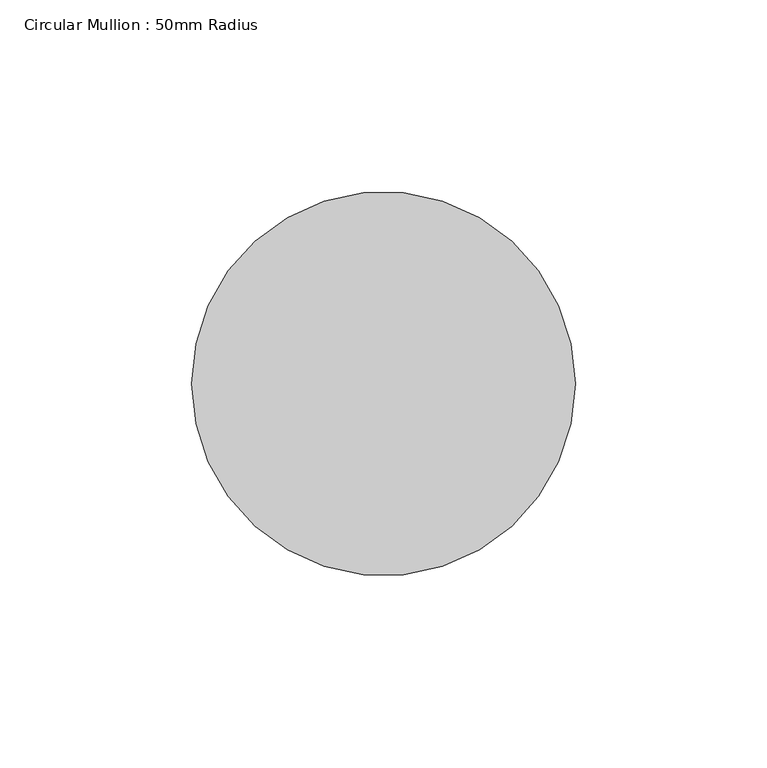
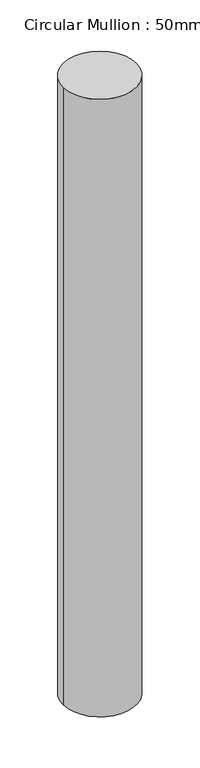
"""IFC4 building model written with IfcOpenShell, lengths in millimetres: member geometry, Circular Mullion : 50mm Radius."""

from ifc_helpers import new_model, si_unit, point, frame, origin, origin_2d, place, context, project, spatial, circle_curve, trimmed, segment, composite_curve, outline, extrude, source, transform, mapped, element, save


def circular_mullion_50mm_radius_6add7e37(model_context):
    return source(origin(), model_context, "Body", "SweptSolid", [
        extrude(outline(composite_curve([segment(trimmed(circle_curve(origin_2d(), 50.0), [point((50.0, 0.0))], [point((-50.0, 0.0))], False, "CARTESIAN"), True, "CONTINUOUS"), segment(trimmed(circle_curve(origin_2d(), 50.0), [point((-50.0, 0.0))], [point((50.0, 0.0))], False, "CARTESIAN"), True, "CONTINUOUS")], self_intersect=False)), frame((0.0, 0.0, -893.5976077), z_axis=(0.0, 0.0, 1.0), x_axis=(1.0, 0.0, 0.0)), (0.0, 0.0, 1.0), 893.5976077),
    ])


if __name__ == "__main__":
    model = new_model("IFC4")
    model_context = context("Model", 3, world=origin())
    ifc_project = project(units=[si_unit("LENGTHUNIT", "METRE", prefix="MILLI")], contexts=[model_context])
    site = spatial("IfcSite", under=ifc_project)
    building = spatial("IfcBuilding", under=site)
    placement = place(None, origin())
    circular_mullion_50mm_radius_shape = circular_mullion_50mm_radius_6add7e37(model_context)
    element("IfcMember", 1, ObjectType="Circular Mullion : 50mm Radius", at=placement, inside=building, context=model_context, shape_type="MappedRepresentation", body=[
        mapped(circular_mullion_50mm_radius_shape, transform((0.0, 0.0, 0.0), x_axis=(1.0, 0.0, 0.0), y_axis=(0.0, 1.0, 0.0), z_axis=(0.0, 0.0, 1.0))),
    ])
    save(model, "model.ifc")

# Revit data of these elements
# Type "Circular Mullion : 50mm Radius"
#   built-in parameter 1007350 = 0.164042 (stored number, unit not read)
# Element 1 (IfcMember, "Circular Mullion : 50mm Radius")
#   Materials on its faces: "Aluminium"
# Materials
#   "Aluminium": class "Metal", colour RGB 247 247 247, transparency 0, Description = "Aluminium 6061", Cost = 0
